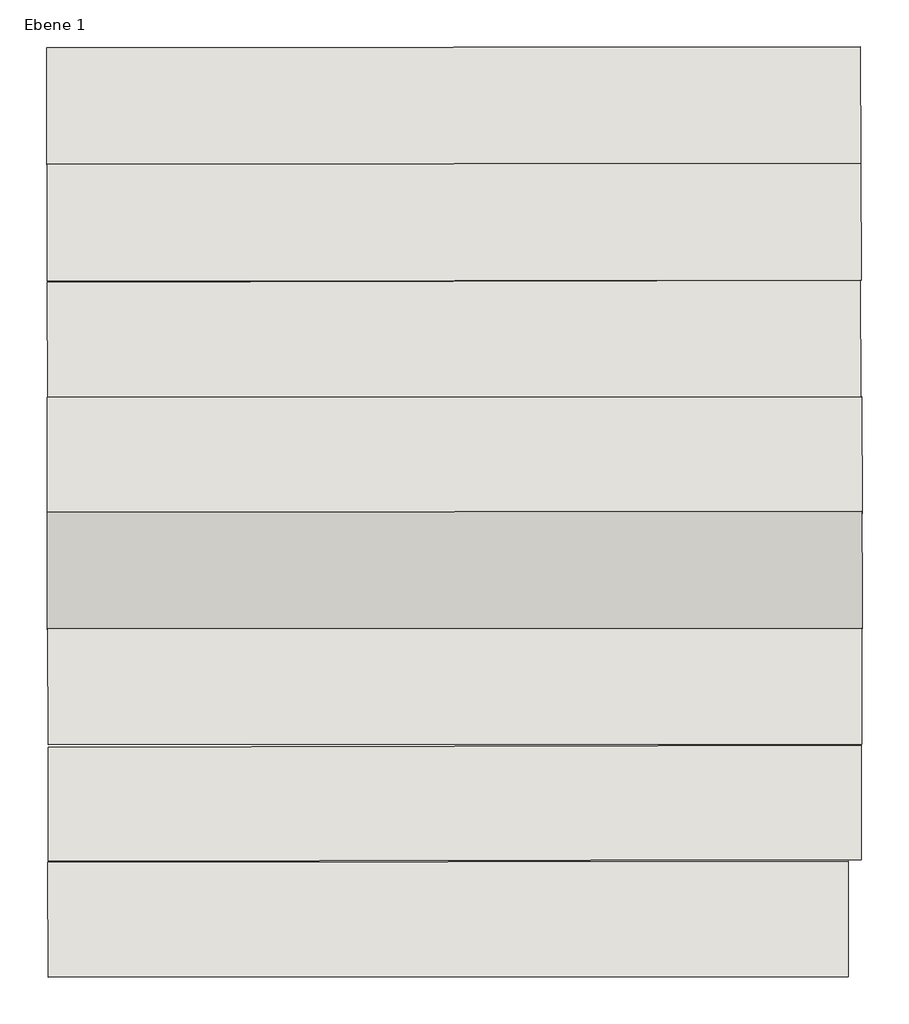
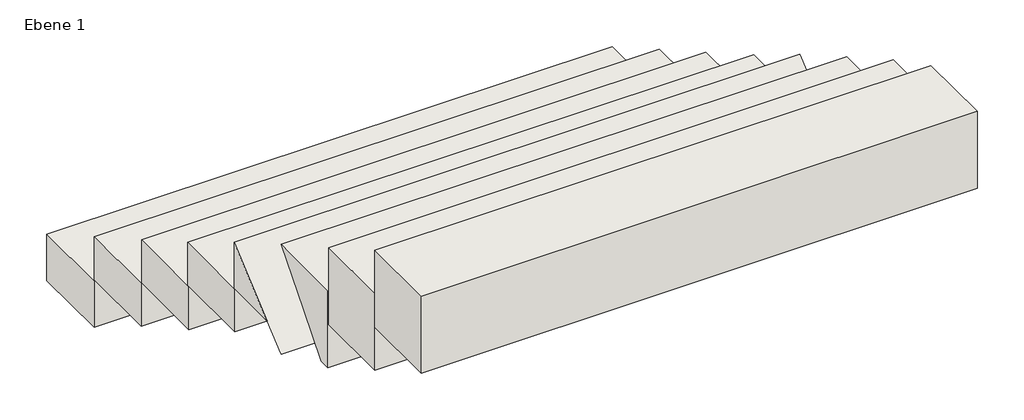
# One storey: 8 walls.
"""IFC4 building model written with IfcOpenShell, lengths in millimetres."""

from ifc_helpers import new_model, si_unit, frame, origin, place, context, project, spatial, polyline, outline, extrude, faceted_brep, element, save

model = new_model("IFC4")

# Units and contexts
model_context = context("Model", 3, world=origin())
ifc_project = project(units=[si_unit("LENGTHUNIT", "METRE", prefix="MILLI")], contexts=[model_context])

# Site, building, storey
site = spatial("IfcSite", under=ifc_project)
building = spatial("IfcBuilding", under=site)
storey = spatial("IfcBuildingStorey", under=building, Name="Ebene 1", Elevation=3040.0)

# Walls
placement = place(None, origin())
element("IfcWall", 1, ObjectType="STB 29.3 - Sichtbeton 10", at=placement, inside=storey, context=model_context, shape_type="SweptSolid", body=[
    extrude(outline(polyline([(4981.7719966, 8163.6090663), (7017.5144154, 8166.1825049), (7018.574112, 7873.1836103), (4982.1423857, 7870.6093004), (4981.7719966, 8163.6090663)])), frame((0.0, 0.0, -1562.973737), z_axis=(0.0, 0.0, 1.0), x_axis=(1.0, 0.0, 0.0)), (0.0, 0.0, 1.0), 175.9923773),
])
element("IfcWall", 2, ObjectType="STB 29.3 - Sichtbeton 10", at=placement, inside=storey, context=model_context, shape_type="SweptSolid", body=[
    extrude(outline(polyline([(4983.3338198, 7872.3394564), (7018.5710788, 7874.0222629), (7019.6307766, 7581.0230389), (4983.5760826, 7579.3395565), (4983.3338198, 7872.3394564)])), frame((0.0, 0.0, -1383.5245183), z_axis=(0.0, 0.0, 1.0), x_axis=(1.0, 0.0, 0.0)), (0.0, 0.0, 1.0), 163.9980712),
])
element("IfcWall", 3, ObjectType="STB 29.3 - Sichtbeton 10", at=placement, inside=storey, context=model_context, shape_type="SweptSolid", body=[
    extrude(outline(polyline([(4983.5859086, 7576.8252914), (7017.468916, 7581.3624158), (7018.1225299, 7288.3631448), (4984.2395225, 7283.8260205), (4983.5859086, 7576.8252914)])), frame((0.0, 0.0, -1216.8129704), z_axis=(0.0, 0.0, 1.0), x_axis=(1.0, 0.0, 0.0)), (0.0, 0.0, 1.0), 163.9983123),
])
element("IfcWall", 4, ObjectType="STB 29.3 - Sichtbeton 10", at=placement, inside=storey, context=model_context, shape_type="SweptSolid", body=[
    extrude(outline(polyline([(4983.2661156, 7288.487656), (7020.681252, 7290.5737533), (7021.7409492, 6997.5746847), (4983.5661164, 6995.4878096), (4983.2661156, 7288.487656)])), frame((0.0, 0.0, -1049.5994694), z_axis=(0.0, 0.0, 1.0), x_axis=(1.0, 0.0, 0.0)), (0.0, 0.0, 1.0), 161.9980581),
])
element("IfcWall", 5, ObjectType="STB 29.3 - Sichtbeton 10", at=placement, inside=storey, context=model_context, shape_type="Brep", body=[
    faceted_brep([(7021.4204399, 7003.0655699, -887.6014138), (4983.5609953, 7000.4894149, -887.6014109), (4983.5609993, 7000.489415, -711.609034), (7021.420446, 7003.0655699, -711.6090392), (7021.7908348, 6710.065804, -887.6014138), (7021.7908323, 6710.065804, -961.6091199), (4983.9313886, 6707.4896491, -961.6091147), (4983.9313902, 6707.4896491, -887.6014109), (7021.6811865, 6796.8027382, -887.6014138), (4983.821742, 6794.2265806, -887.6014109), (4983.9275934, 6710.4918593, -959.047499), (7021.7870371, 6713.0680143, -959.0475042)], [[[0, 1, 2, 3]], [[4, 5, 6, 7]], [[1, 0, 8, 4, 7, 9]], [[2, 1, 9]], [[0, 3, 8]], [[3, 2, 9, 10, 6, 5, 11, 8]], [[9, 7, 6, 10]], [[8, 11, 5, 4]]]),
])
element("IfcWall", 6, ObjectType="STB 29.3 - Sichtbeton 10", at=placement, inside=storey, context=model_context, shape_type="Brep", body=[
    faceted_brep([(4985.4942097, 6419.225298, -837.1542814), (4985.4520848, 6459.2206395, -837.1542704), (7021.3652019, 6460.9040488, -837.1542758), (7021.4073268, 6420.9087072, -837.1542868), (4985.4942106, 6419.2252173, -544.1542814), (7021.4073276, 6420.9086266, -544.1542868), (7021.1018918, 6710.9039166, -544.154207), (4985.1887747, 6709.2205073, -544.1542015), (7021.2492718, 6570.9739316, -708.1522747), (4985.3361547, 6569.2905223, -708.1522692)], [[[0, 1, 2, 3]], [[4, 5, 6, 7]], [[5, 4, 0, 3]], [[6, 5, 3, 2, 8]], [[4, 7, 9, 1, 0]], [[7, 6, 8, 2, 1, 9]]]),
])
element("IfcWall", 7, ObjectType="STB 29.3 - Sichtbeton 10", at=placement, inside=storey, context=model_context, shape_type="SweptSolid", body=[
    extrude(outline(polyline([(13912.305652, 31722.5696836), (13653.4475619, 31600.9678087), (12789.0836076, 33442.0520496), (13047.9416977, 33563.6539244), (13912.305652, 31722.5696836)])), frame((-17874.7972917, 32151.6994647, -670.4353405), z_axis=(2.9007046162432886e-09, -2.753599033385781e-07, 0.9999999999999621), x_axis=(-0.4229599190653321, -0.9061483911943927, -2.4829005161998675e-07)), (0.0, 0.0, 1.0), 293.0),
])
element("IfcWall", 8, ObjectType="STB 29.3 - Sichtbeton 10", at=placement, inside=storey, context=model_context, shape_type="SweptSolid", body=[
    extrude(outline(polyline([(14175.6474351, 31844.8298439), (13914.8312226, 31722.692135), (13066.2335644, 33535.8795142), (13327.0497768, 33658.0172232), (14175.6474351, 31844.8298439)])), frame((-17874.7972913, 32151.6994192, -505.2220936), z_axis=(2.9007047280758045e-09, -2.7535990323852005e-07, 0.9999999999999621), x_axis=(-0.4229599190653321, -0.9061483911943927, -2.4829005148201864e-07)), (0.0, 0.0, 1.0), 293.0),
])

save(model, "model.ifc")

# Revit data of these elements
# Type "STB 29.3 - Sichtbeton 10"
#   Type Comments = "Stahlbeton Sichtbeton"
#   Description = "Stahlbeton (Sichtbeton) 30.0"
#   Layers, outside or top first: 0.293 m "Stahlbeton - Sichtbeton (1)" (function 1)
# Element 1 (IfcWall, "STB 29.3 - Sichtbeton 10")
#   built-in parameter 1001111 = -4.602974 m
#   Top Offset = 0.000 m
#   Base Offset = -4.602974 m
#   Unconnected Height = 0.175992 m
#   wall height = 0.175992 m
#   Phase Created = Phase 1
#   Base Constraint = Ebene 1
#   Materials on its faces: "Stahlbeton - Sichtbeton (1)"
# Element 2 (IfcWall, "STB 29.3 - Sichtbeton 10")
#   built-in parameter 1001111 = -4.423525 m
#   Top Offset = 0.000 m
#   Base Offset = -4.423525 m
#   Unconnected Height = 0.163998 m
#   wall height = 0.163998 m
#   Phase Created = Phase 1
#   Base Constraint = Ebene 1
#   Materials on its faces: "Stahlbeton - Sichtbeton (1)"
# Element 3 (IfcWall, "STB 29.3 - Sichtbeton 10")
#   built-in parameter 1001111 = -4.256813 m
#   Top Offset = 0.000 m
#   Base Offset = -4.256813 m
#   Unconnected Height = 0.163998 m
#   wall height = 0.163998 m
#   Phase Created = Phase 1
#   Base Constraint = Ebene 1
#   Materials on its faces: "Stahlbeton - Sichtbeton (1)"
# Element 4 (IfcWall, "STB 29.3 - Sichtbeton 10")
#   built-in parameter 1001111 = -4.089599 m
#   Top Offset = 0.000 m
#   Base Offset = -4.089599 m
#   Unconnected Height = 0.161998 m
#   wall height = 0.161998 m
#   Phase Created = Phase 1
#   Base Constraint = Ebene 1
#   Materials on its faces: "Stahlbeton - Sichtbeton (1)"
# Element 5 (IfcWall, "STB 29.3 - Sichtbeton 10")
#   built-in parameter 1001111 = -3.927601 m
#   Top Offset = 0.000 m
#   Base Offset = -3.927601 m
#   Unconnected Height = 0.175992 m
#   wall height = 0.175992 m
#   Phase Created = Phase 1
#   Base Constraint = Ebene 1
#   Materials on its faces: "Stahlbeton - Sichtbeton (1)"
# Elements 6, 7, 8 (IfcWall, "STB 29.3 - Sichtbeton 10")
#   Phase Created = Phase 1
#   Materials on its faces: "Stahlbeton - Sichtbeton (1)"
# Materials
#   "Stahlbeton - Sichtbeton (1)": class "Beton", colour RGB 192 192 192, transparency 0, Cost = 0
